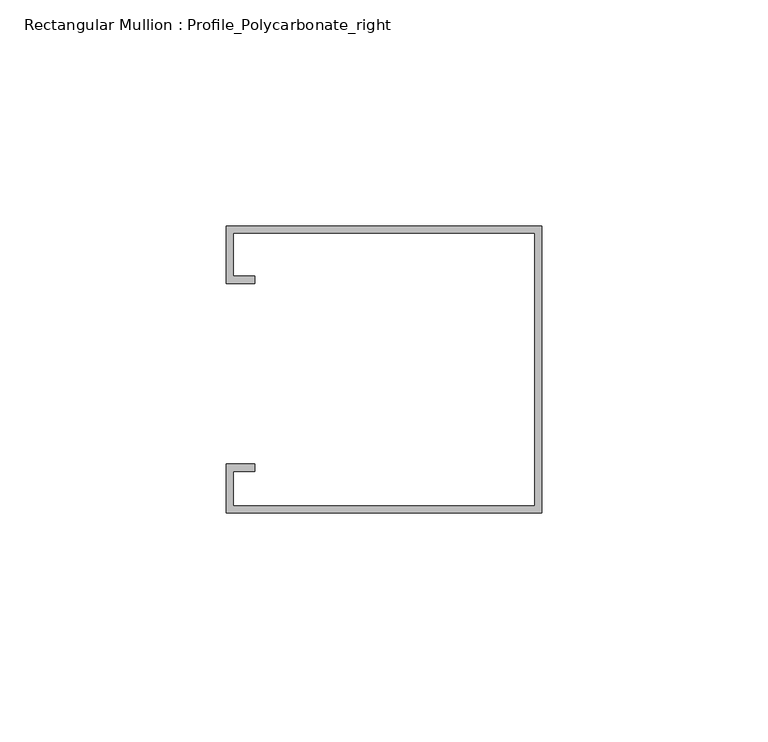
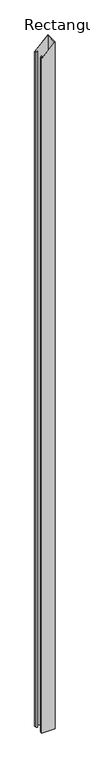
"""IFC4 building model written with IfcOpenShell, lengths in millimetres: member geometry, Rectangular Mullion : Profile_Polycarbonate_right."""

import ifcopenshell
import ifcopenshell.guid

model = None  # the IFC model being written
_history = None  # IfcOwnerHistory: only IFC2X3 demands one
_inside = {}  # id of a spatial element -> (the spatial element, [elements in it])
_under = {}  # id of a project, library or spatial element -> (it, [spatial elements below it])
_declared = {}  # id of a project -> (the project, [libraries it declares])
_typed = {}  # id of a type object -> (the type object, [elements of that type])
_made_of = {}  # id of a material, layer set ... -> (it, [elements and type objects made of it])


def new_model(schema):
    """Start an empty IFC model of exactly this schema.

    Asked for "IFC4X3", IfcOpenShell would pick the latest addendum, in which some entities
    have other attributes; the version numbers below select the first issue.
    IFC2X3 requires an IfcOwnerHistory on every rooted entity: one is made here for all.
    """
    global model, _history
    if schema == "IFC4X3":
        model = ifcopenshell.file(schema_version=(4, 3, 0, 0))
    else:
        model = ifcopenshell.file(schema=schema)
    _inside.clear()
    _under.clear()
    _declared.clear()
    _typed.clear()
    _made_of.clear()
    _history = None
    if model.schema == "IFC2X3":
        org = make("IfcOrganization", Name="unknown")
        user = make(
            "IfcPersonAndOrganization",
            ThePerson=make("IfcPerson", FamilyName="unknown"),
            TheOrganization=org,
        )
        app = make(
            "IfcApplication",
            ApplicationDeveloper=org,
            Version="unknown",
            ApplicationFullName="unknown",
            ApplicationIdentifier="unknown",
        )
        _history = make(
            "IfcOwnerHistory",
            OwningUser=user,
            OwningApplication=app,
            ChangeAction="ADDED",
            CreationDate=0,
        )
    return model


def make(cls, **values):
    """One entity of the class cls with the attributes given. An attribute that is None is left unset."""
    return model.create_entity(
        cls, **{name: value for name, value in values.items() if value is not None}
    )


def rooted(cls, **values):
    """An entity with a GlobalId (a new one), such as an element, a storey or a relation."""
    return make(cls, GlobalId=ifcopenshell.guid.new(), OwnerHistory=_history, **values)


def si_unit(unit_type, name, prefix=None):
    """IfcSIUnit, for example si_unit("LENGTHUNIT", "METRE", prefix="MILLI")."""
    return make("IfcSIUnit", UnitType=unit_type, Prefix=prefix, Name=name)


def assignment(units):
    """IfcUnitAssignment: the units of a project."""
    return None if units is None else make("IfcUnitAssignment", Units=units)


def point(xyz):
    """IfcCartesianPoint."""
    return None if xyz is None else make("IfcCartesianPoint", Coordinates=xyz)


def direction(xyz):
    """IfcDirection."""
    return None if xyz is None else make("IfcDirection", DirectionRatios=xyz)


def frame(location, z_axis=None, x_axis=None):
    """IfcAxis2Placement3D, a coordinate frame: its origin and axes. An axis left out is left unset."""
    return make(
        "IfcAxis2Placement3D",
        Location=point(location),
        Axis=direction(z_axis),
        RefDirection=direction(x_axis),
    )


def origin():
    """The frame at (0, 0, 0) with its axes left unset."""
    return frame((0.0, 0.0, 0.0))


def place(relative_to, where):
    """IfcLocalPlacement: puts the frame where relative to a parent placement (None: the world)."""
    return make(
        "IfcLocalPlacement", PlacementRelTo=relative_to, RelativePlacement=where
    )


def context(
    kind, dimensions, precision=None, world=None, true_north=None, identifier=None
):
    """IfcGeometricRepresentationContext, for example the 3D "Model" context."""
    return make(
        "IfcGeometricRepresentationContext",
        ContextIdentifier=identifier,
        ContextType=kind,
        CoordinateSpaceDimension=dimensions,
        Precision=precision,
        WorldCoordinateSystem=world,
        TrueNorth=true_north,
    )


def project(units=None, contexts=None):
    """IfcProject with its units and contexts."""
    return rooted(
        "IfcProject",
        Name="project",
        RepresentationContexts=contexts,
        UnitsInContext=assignment(units),
    )


def spatial(cls, under=None, at=None, **own):
    """A site, building, storey or space (cls), placed at a placement, below another one or the project."""
    s = rooted(cls, ObjectPlacement=at, **own)
    if under is not None:
        _under.setdefault(under.id(), (under, []))[1].append(s)
    return s


def faces_of(points, faces, orient=None, outer=None):
    """IfcFace entities. A face is a list of loops; a loop is a list of indices into points, from 0.

    orient and outer hold one flag for each loop. By default every Orientation is true, the
    first loop of a face is its IfcFaceOuterBound and the others are IfcFaceBound.
    """
    made = []
    for i, loops in enumerate(faces):
        bounds = []
        for j, loop in enumerate(loops):
            is_outer = j == 0 if outer is None else outer[i][j]
            bounds.append(
                make(
                    "IfcFaceOuterBound" if is_outer else "IfcFaceBound",
                    Bound=make("IfcPolyLoop", Polygon=[points[k] for k in loop]),
                    Orientation=True if orient is None else orient[i][j],
                )
            )
        made.append(make("IfcFace", Bounds=bounds))
    return made


def faceted_brep(points, faces, orient=None, outer=None, voids=None):
    """IfcFacetedBrep: a solid bounded by flat faces; with voids (closed shells), ...WithVoids."""
    shared = [point(p) for p in points]
    hull = make("IfcClosedShell", CfsFaces=faces_of(shared, faces, orient, outer))
    if voids is None:
        return make("IfcFacetedBrep", Outer=hull)
    return make(
        "IfcFacetedBrepWithVoids",
        Outer=hull,
        Voids=[
            make(cls, CfsFaces=faces_of(shared, fs, o, b)) for cls, fs, o, b in voids
        ],
    )


def shape(context_of_items, identifier, shape_type, items):
    """IfcShapeRepresentation: the items that make up one representation, for example the "Body"."""
    return make(
        "IfcShapeRepresentation",
        ContextOfItems=context_of_items,
        RepresentationIdentifier=identifier,
        RepresentationType=shape_type,
        Items=items,
    )


def source(mapping_origin, context_of_items, identifier, shape_type, items):
    """IfcRepresentationMap: a shape defined once, which mapped items show again and again."""
    return make(
        "IfcRepresentationMap",
        MappingOrigin=mapping_origin,
        MappedRepresentation=shape(context_of_items, identifier, shape_type, items),
    )


def transform(
    local_origin,
    x_axis=None,
    y_axis=None,
    z_axis=None,
    scale=None,
    scale2=None,
    scale3=None,
    uniform=True,
):
    """IfcCartesianTransformationOperator3D, or its non-uniform kind. x_axis, y_axis, z_axis: its Axis1, 2, 3."""
    if uniform:
        return make(
            "IfcCartesianTransformationOperator3D",
            Axis1=direction(x_axis),
            Axis2=direction(y_axis),
            LocalOrigin=point(local_origin),
            Scale=scale,
            Axis3=direction(z_axis),
        )
    return make(
        "IfcCartesianTransformationOperator3DnonUniform",
        Axis1=direction(x_axis),
        Axis2=direction(y_axis),
        LocalOrigin=point(local_origin),
        Scale=scale,
        Axis3=direction(z_axis),
        Scale2=scale2,
        Scale3=scale3,
    )


def mapped(mapping_source, mapping_target):
    """IfcMappedItem: shows the shape of a source again, moved by a transform."""
    return make(
        "IfcMappedItem", MappingSource=mapping_source, MappingTarget=mapping_target
    )


def made_of(thing, what):
    """Note that an element or type object is made of a material, layer set ...; save() writes the relation."""
    if what is not None:
        _made_of.setdefault(what.id(), (what, []))[1].append(thing)
    return thing


def element(
    cls,
    number,
    at=None,
    inside=None,
    cuts=None,
    type_object=None,
    material=None,
    context=None,
    identifier="Body",
    shape_type=None,
    held_by="IfcProductDefinitionShape",
    body=None,
    shapes=None,
    **own,
):
    """One element of the class cls, such as IfcWall. Its Tag is "e" and its number.

    at: its placement. inside: the storey or other place that contains it. cuts: it is an
    opening in that element (IfcRelVoidsElement). A single representation is given by context,
    identifier, shape_type and body (its items); several are given by shapes. held_by: the class
    of the entity that holds the representations. save() writes the other relations.
    """
    e = rooted(cls, Tag="e%d" % number, ObjectPlacement=at, **own)
    if body is not None:
        shapes = [shape(context, identifier, shape_type, body)]
    if shapes is not None:
        e.Representation = make(held_by, Representations=shapes)
    if inside is not None:
        _inside.setdefault(inside.id(), (inside, []))[1].append(e)
    if cuts is not None:
        rooted(
            "IfcRelVoidsElement", RelatingBuildingElement=cuts, RelatedOpeningElement=e
        )
    if type_object is not None:
        _typed.setdefault(type_object.id(), (type_object, []))[1].append(e)
    return made_of(e, material)


def aggregate(whole, parts):
    """IfcRelAggregates: a whole, such as a stair, and the parts it consists of."""
    return rooted("IfcRelAggregates", RelatingObject=whole, RelatedObjects=parts)


def save(model, path):
    """Write the relations noted so far, then the file.

    IfcRelAggregates (storeys below a building ...), IfcRelContainedInSpatialStructure (elements
    in a storey), IfcRelDefinesByType, IfcRelAssociatesMaterial and IfcRelDeclares: one each for
    every whole, place, type object, material and project.
    """
    for whole, parts in _under.values():
        aggregate(whole, parts)
    for where, things in _inside.values():
        rooted(
            "IfcRelContainedInSpatialStructure",
            RelatedElements=things,
            RelatingStructure=where,
        )
    for kind, things in _typed.values():
        rooted("IfcRelDefinesByType", RelatedObjects=things, RelatingType=kind)
    for what, things in _made_of.values():
        rooted("IfcRelAssociatesMaterial", RelatedObjects=things, RelatingMaterial=what)
    for by, libraries in _declared.values():
        rooted("IfcRelDeclares", RelatingContext=by, RelatedDefinitions=libraries)
    model.write(path)


def rectangular_mullion_profile_polycarbonate_right_f9876bef(model_context):
    return source(origin(), model_context, "Body", "Brep", [
        faceted_brep([(0.0, 32.7, -3772.1642939), (0.0, -30.8, -3772.1642939), (-69.85, -30.8, -3772.1642939), (-69.85, -20.0, -3772.1642939), (-63.5, -20.0, -3772.1642939), (-63.5, -21.5875, -3772.1642939), (-68.2625, -21.5875, -3772.1642939), (-68.2625, -29.2125, -3772.1642939), (-1.5875, -29.2125, -3772.1642939), (-1.5875, 31.1125, -3772.1642939), (-68.2625, 31.1125, -3772.1642939), (-68.2625, 21.5875, -3772.1642939), (-63.5, 21.5875, -3772.1642939), (-63.5, 20.0, -3772.1642939), (-69.85, 20.0, -3772.1642939), (-69.85, 32.7, -3772.1642939), (-69.85, 32.7, -67.0001907), (0.0, 32.7, 0.0), (-69.85, 20.0, -67.0001907), (-63.5, 20.0, -60.9092643), (-63.5, 21.5875, -60.9092643), (-68.2625, 21.5875, -65.4774591), (-68.2625, 31.1125, -65.4774591), (-1.5875, 31.1125, -1.5227316), (-1.5875, -29.2125, -1.5227316), (-68.2625, -29.2125, -65.4774591), (-68.2625, -21.5875, -65.4774591), (-63.5, -21.5875, -60.9092643), (-63.5, -20.0, -60.9092643), (-69.85, -20.0, -67.0001907), (-69.85, -30.8, -67.0001907), (0.0, -30.8, 0.0)], [[[0, 1, 2, 3, 4, 5, 6, 7, 8, 9, 10, 11, 12, 13, 14, 15]], [[16, 17, 0, 15]], [[18, 16, 15, 14]], [[19, 18, 14, 13]], [[20, 19, 13, 12]], [[21, 20, 12, 11]], [[22, 21, 11, 10]], [[23, 22, 10, 9]], [[24, 23, 9, 8]], [[25, 24, 8, 7]], [[26, 25, 7, 6]], [[27, 26, 6, 5]], [[28, 27, 5, 4]], [[29, 28, 4, 3]], [[30, 29, 3, 2]], [[31, 30, 2, 1]], [[17, 31, 1, 0]], [[17, 16, 18, 19, 20, 21, 22, 23, 24, 25, 26, 27, 28, 29, 30, 31]]]),
    ])


if __name__ == "__main__":
    model = new_model("IFC4")
    model_context = context("Model", 3, world=origin())
    ifc_project = project(units=[si_unit("LENGTHUNIT", "METRE", prefix="MILLI")], contexts=[model_context])
    site = spatial("IfcSite", under=ifc_project)
    building = spatial("IfcBuilding", under=site)
    placement = place(None, origin())
    rectangular_mullion_profile_polycarbonate_right_shape = rectangular_mullion_profile_polycarbonate_right_f9876bef(model_context)
    element("IfcMember", 1, ObjectType="Rectangular Mullion : Profile_Polycarbonate_right", at=placement, inside=building, context=model_context, shape_type="MappedRepresentation", body=[
        mapped(rectangular_mullion_profile_polycarbonate_right_shape, transform((0.0, 0.0, 0.0), x_axis=(1.0, 0.0, 0.0), y_axis=(0.0, 1.0, 0.0), z_axis=(0.0, 0.0, 1.0))),
    ])
    save(model, "model.ifc")

# Revit data of these elements
# Type "Rectangular Mullion : Profile_Polycarbonate_right"
#   built-in parameter 1007322 = 0.208333 (stored number, unit not read)
#   built-in parameter 1007321 = 0 (stored number, unit not read)
#   built-in parameter 1007320 = 0.00520833 (stored number, unit not read)
